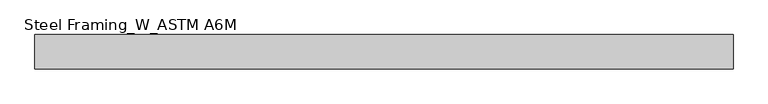
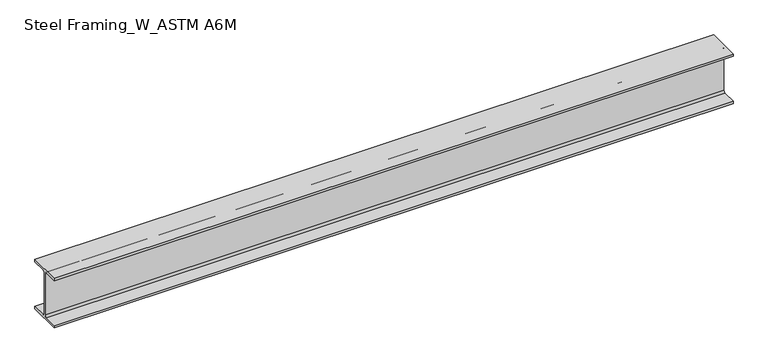
"""IFC4 building model written with IfcOpenShell, lengths in millimetres: beam geometry, Steel Framing_W_ASTM A6M : H_SB_AR_S02_W200x31.3_B6."""

from ifc_helpers import new_model, si_unit, point, frame, frame_2d, origin, place, context, project, spatial, polyline, circle_curve, trimmed, segment, composite_curve, outline, extrude, source, transform, mapped, element, save


def steel_framing_w_astm_a6m_9acaacfc(model_context):
    return source(origin(), model_context, "Body", "SweptSolid", [
        extrude(outline(composite_curve([segment(polyline([(67.0, -94.8), (67.0, -105.0), (-67.0, -105.0), (-67.0, -94.8), (-10.775, -94.8)]), True, "CONTINUOUS"), segment(trimmed(circle_curve(frame_2d((-10.775, -87.2)), 7.6), [point((-10.775, -94.8))], [point((-3.175, -87.2))], True, "CARTESIAN"), True, "CONTINUOUS"), segment(polyline([(-3.175, -87.2), (-3.175, 87.2)]), True, "CONTINUOUS"), segment(trimmed(circle_curve(frame_2d((-10.775, 87.2)), 7.6), [point((-3.175, 87.2))], [point((-10.775, 94.8))], True, "CARTESIAN"), True, "CONTINUOUS"), segment(polyline([(-10.775, 94.8), (-67.0, 94.8), (-67.0, 105.0), (67.0, 105.0), (67.0, 94.8), (10.775, 94.8)]), True, "CONTINUOUS"), segment(trimmed(circle_curve(frame_2d((10.775, 87.2)), 7.6), [point((10.775, 94.8))], [point((3.175, 87.2))], True, "CARTESIAN"), True, "CONTINUOUS"), segment(polyline([(3.175, 87.2), (3.175, -87.2)]), True, "CONTINUOUS"), segment(trimmed(circle_curve(frame_2d((10.775, -87.2)), 7.6), [point((3.175, -87.2))], [point((10.775, -94.8))], True, "CARTESIAN"), True, "CONTINUOUS"), segment(polyline([(10.775, -94.8), (67.0, -94.8)]), True, "CONTINUOUS")], self_intersect=False)), frame((-1360.3, 0.0, 0.0), z_axis=(1.0, 0.0, 0.0), x_axis=(0.0, 1.0, 0.0)), (0.0, 0.0, 1.0), 2720.6),
    ])


if __name__ == "__main__":
    model = new_model("IFC4")
    model_context = context("Model", 3, world=origin())
    ifc_project = project(units=[si_unit("LENGTHUNIT", "METRE", prefix="MILLI")], contexts=[model_context])
    site = spatial("IfcSite", under=ifc_project)
    building = spatial("IfcBuilding", under=site)
    placement = place(None, origin())
    steel_framing_w_astm_a6m_shape = steel_framing_w_astm_a6m_9acaacfc(model_context)
    element("IfcBeam", 1, ObjectType="Steel Framing_W_ASTM A6M : H_SB_AR_S02_W200x31.3_B6", at=placement, inside=building, context=model_context, shape_type="MappedRepresentation", body=[
        mapped(steel_framing_w_astm_a6m_shape, transform((0.0, 0.0, 0.0), x_axis=(1.0, 0.0, 0.0), y_axis=(0.0, 1.0, 0.0), z_axis=(0.0, 0.0, 1.0))),
    ])
    save(model, "model.ifc")

# Revit data of these elements
# Type "Steel Framing_W_ASTM A6M : H_SB_AR_S02_W200x31.3_B6"
#   Type Mark = "B6"
#   Section Name Key = "W8x21"
#   Width = 13.4 cm
#   Web Thickness = 0.635 cm
#   Web Fillet = 0.76 cm
#   Warping Constant = 40800.0 cm⁶
#   Torsional Moment of Inertia = 11.70 cm⁴
#   Section Area = 39.7 cm²
#   Plastic Modulus weak axis = 93.2 cm³
#   Plastic Modulus strong axis = 334.0 cm³
#   Perimeter = 0.93 m²/m
#   Nominal Weight = 31.30 kgf/m
#   Moment of Inertia weak axis = 407.00 cm⁴
#   Moment of Inertia strong axis = 3130.00 cm⁴
#   Height = 21.0 cm
#   Flange Thickness = 1.02 cm
#   Elastic Modulus weak axis = 60.8 cm³
#   Elastic Modulus strong axis = 298.0 cm³
#   Centroid Vertical = 10.5 cm
#   Centroid Horizontal = 6.7 cm
#   Length [instance default] = 1500 mm
#   Structural Material [instance default] = Steel, 45-345
#   Bolt Spacing = 0
#   Assembly Code = ""
# Element 1 (IfcBeam, "Steel Framing_W_ASTM A6M : H_SB_AR_S02_W200x31.3_B6")
#   Materials on its faces: "Steel, 45-345"
# Materials
#   "Steel, 45-345": class "Metal", colour RGB 189 187 185, transparency 0, Description = "Steel 345 MPa", Cost = 0
